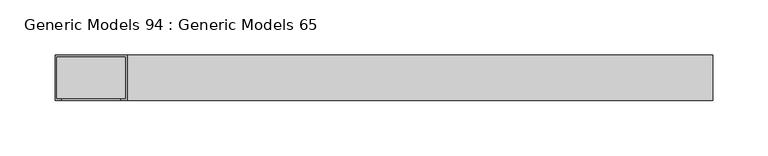
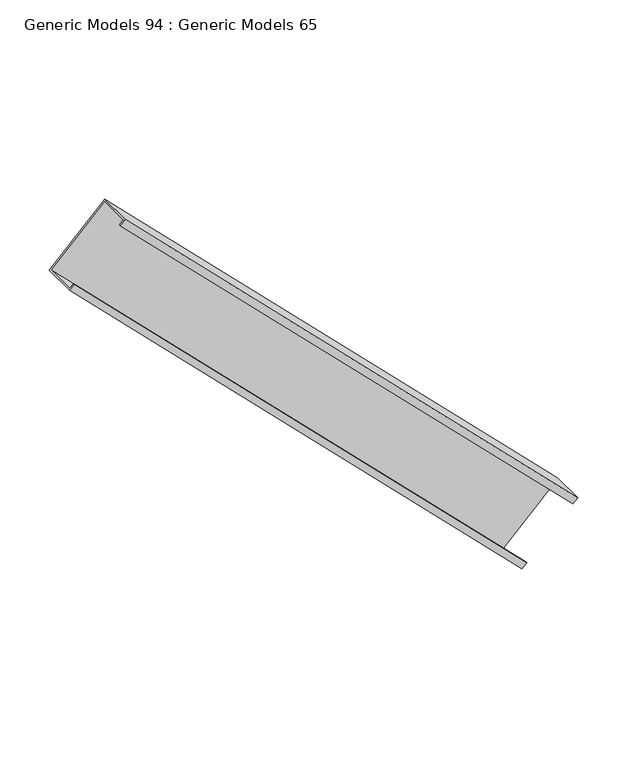
"""IFC4 building model written with IfcOpenShell, lengths in millimetres: proxy geometry, Generic Models 94 : Generic Models 65."""

from ifc_helpers import new_model, si_unit, frame, origin, place, context, project, spatial, polyline, outline, extrude, source, transform, mapped, element, save


def generic_models_94_generic_models_65_014fd4cc(model_context):
    return source(origin(), model_context, "Body", "SweptSolid", [
        extrude(outline(polyline([(0.0, -92.075), (0.0, 0.0), (41.275, 0.0), (41.275, -7.9375), (39.6875, -7.9375), (39.6875, -1.5875), (1.5875, -1.5875), (1.5875, -90.4875001), (39.6875, -90.4875001), (39.6875, -84.1375), (41.275, -84.1375), (41.275, -92.075), (0.0, -92.075)])), frame((51013.5806639, 630.2375, -131.5464946), z_axis=(-0.7071067811865384, 0.0, 0.7071067811865568), x_axis=(0.0, -1.0, 0.0)), (0.0, 0.0, 1.0), 749.9641452),
    ])


if __name__ == "__main__":
    model = new_model("IFC4")
    model_context = context("Model", 3, world=origin())
    ifc_project = project(units=[si_unit("LENGTHUNIT", "METRE", prefix="MILLI")], contexts=[model_context])
    site = spatial("IfcSite", under=ifc_project)
    building = spatial("IfcBuilding", under=site)
    placement = place(None, origin())
    generic_models_94_generic_models_65_shape = generic_models_94_generic_models_65_014fd4cc(model_context)
    element("IfcBuildingElementProxy", 1, Name="Generic Models 94 : Generic Models 65", ObjectType="Generic Models 94 : Generic Models 65", at=placement, inside=building, context=model_context, shape_type="MappedRepresentation", body=[
        mapped(generic_models_94_generic_models_65_shape, transform((0.0, 0.0, 0.0), x_axis=(1.0, 0.0, 0.0), y_axis=(0.0, 1.0, 0.0), z_axis=(0.0, 0.0, 1.0))),
    ])
    save(model, "model.ifc")

# Revit data of these elements
# Element 1 (IfcBuildingElementProxy, "Generic Models 94 : Generic Models 65")
#   Materials on its faces: "DIAGONAL BRACING AS NECESSARY - ATTACH TO STRUCTURAL DECK"
# Materials
#   "DIAGONAL BRACING AS NECESSARY - ATTACH TO STRUCTURAL DECK": class "Unassigned", colour RGB 210 209 208, transparency 0, Keynote = "M05121300.02", Cost = 0
